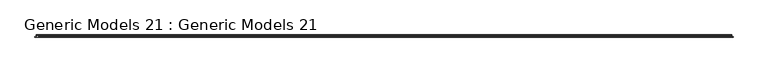
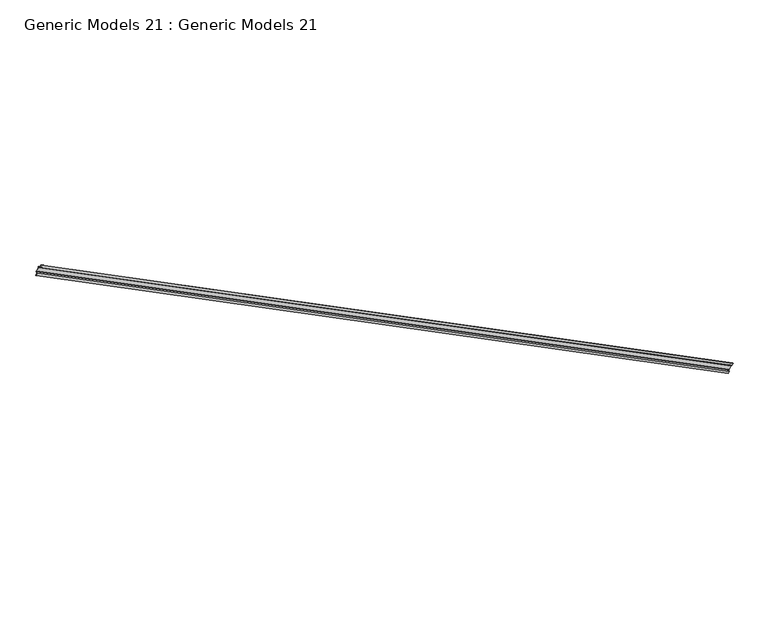
"""IFC4 building model written with IfcOpenShell, lengths in millimetres: proxy geometry, Generic Models 21 : Generic Models 21."""

from ifc_helpers import new_model, si_unit, point, frame, frame_2d, origin, place, context, project, spatial, polyline, circle_curve, trimmed, segment, composite_curve, outline, extrude, source, transform, mapped, element, save


def generic_models_21_generic_models_21_a3cf2a27(model_context):
    return source(origin(), model_context, "Body", "SweptSolid", [
        extrude(outline(composite_curve([segment(polyline([(1.5875, 49.9746691), (10.8316343, 47.9357719)]), True, "CONTINUOUS"), segment(trimmed(circle_curve(frame_2d((10.31875, 45.6104115)), 2.38125), [point((10.8316343, 47.9357719))], [point((11.90625, 43.8355325))], False, "CARTESIAN"), True, "CONTINUOUS"), segment(trimmed(circle_curve(frame_2d((13.49375, 42.0606535)), 2.38125), [point((11.90625, 43.8355325))], [point((11.1125, 42.0606535))], True, "CARTESIAN"), True, "CONTINUOUS"), segment(polyline([(11.1125, 42.0606535), (11.1125, 21.4393466)]), True, "CONTINUOUS"), segment(trimmed(circle_curve(frame_2d((13.49375, 21.4393466)), 2.38125), [point((11.1125, 21.4393466))], [point((11.90625, 19.6644676))], True, "CARTESIAN"), True, "CONTINUOUS"), segment(trimmed(circle_curve(frame_2d((10.31875, 17.8895886)), 2.38125), [point((11.90625, 19.6644676))], [point((10.8316343, 15.5642282))], False, "CARTESIAN"), True, "CONTINUOUS"), segment(polyline([(10.8316343, 15.5642282), (1.5875, 13.525331), (1.5875, 0.0), (0.0, 0.0), (0.0, 14.8008453), (10.4897114, 17.1144685)]), True, "CONTINUOUS"), segment(trimmed(circle_curve(frame_2d((10.31875, 17.8895886)), 0.79375), [point((10.4897114, 17.1144685))], [point((10.8479167, 18.481215))], True, "CARTESIAN"), True, "CONTINUOUS"), segment(trimmed(circle_curve(frame_2d((13.49375, 21.4393466)), 3.96875), [point((10.8479167, 18.481215))], [point((9.525, 21.4393466))], False, "CARTESIAN"), True, "CONTINUOUS"), segment(polyline([(9.525, 21.4393466), (9.525, 42.0606535)]), True, "CONTINUOUS"), segment(trimmed(circle_curve(frame_2d((13.49375, 42.0606535)), 3.96875), [point((9.525, 42.0606535))], [point((10.8479167, 45.0187851))], False, "CARTESIAN"), True, "CONTINUOUS"), segment(trimmed(circle_curve(frame_2d((10.31875, 45.6104115)), 0.79375), [point((10.8479167, 45.0187851))], [point((10.4897114, 46.3855316))], True, "CARTESIAN"), True, "CONTINUOUS"), segment(polyline([(10.4897114, 46.3855316), (0.0, 48.6991548), (0.0, 63.5000001), (1.5875, 63.5000001), (1.5875, 49.9746691)]), True, "CONTINUOUS")], self_intersect=False)), frame((32024.7654415, 40959.4231612, 272160.2011072), z_axis=(-0.8944271909999285, 0.0, 0.4472135954999328), x_axis=(0.0, 1.0, 0.0)), (0.0, 0.0, 1.0), 4676.5930666),
    ])


if __name__ == "__main__":
    model = new_model("IFC4")
    model_context = context("Model", 3, world=origin())
    ifc_project = project(units=[si_unit("LENGTHUNIT", "METRE", prefix="MILLI")], contexts=[model_context])
    site = spatial("IfcSite", under=ifc_project)
    building = spatial("IfcBuilding", under=site)
    placement = place(None, origin())
    generic_models_21_generic_models_21_shape = generic_models_21_generic_models_21_a3cf2a27(model_context)
    element("IfcBuildingElementProxy", 1, Name="Generic Models 21 : Generic Models 21", ObjectType="Generic Models 21 : Generic Models 21", at=placement, inside=building, context=model_context, shape_type="MappedRepresentation", body=[
        mapped(generic_models_21_generic_models_21_shape, transform((0.0, 0.0, 0.0), x_axis=(1.0, 0.0, 0.0), y_axis=(0.0, 1.0, 0.0), z_axis=(0.0, 0.0, 1.0))),
    ])
    save(model, "model.ifc")

# Revit data of these elements
# Element 1 (IfcBuildingElementProxy, "Generic Models 21 : Generic Models 21")
#   Materials on its faces: "1/2\" DEEP GALV. HORTZ. HAT CHANNEL @ XX O.C."
# Materials
#   "1/2\" DEEP GALV. HORTZ. HAT CHANNEL @ XX O.C.": class "Generic", colour RGB 212 212 212, transparency 0, Cost = 0
